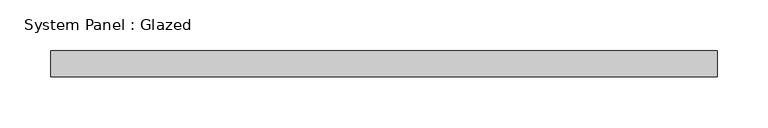
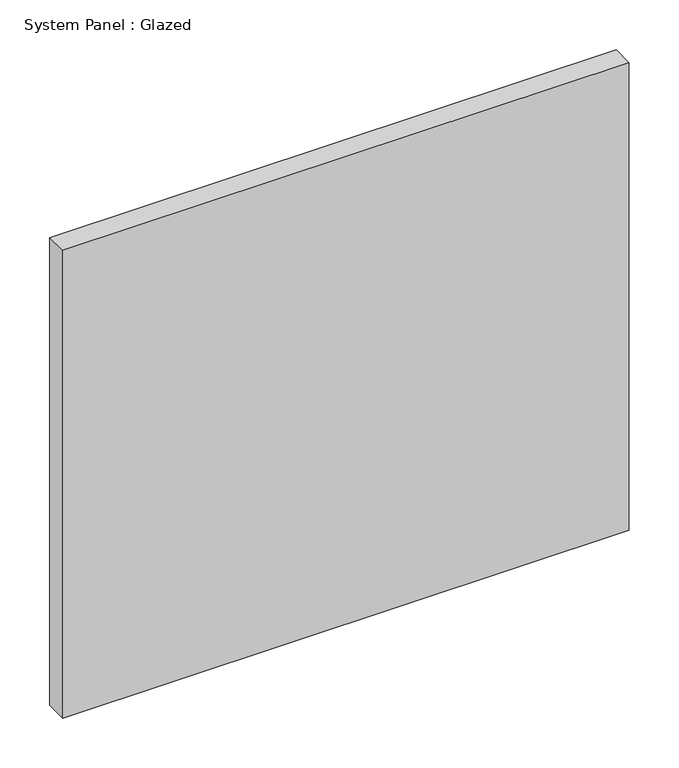
"""IFC4 building model written with IfcOpenShell, lengths in millimetres: plate geometry, System Panel : Glazed."""

from ifc_helpers import new_model, si_unit, origin, origin_with_axes, place, context, project, spatial, polyline, outline, extrude, source, transform, mapped, element, save


def system_panel_glazed_6e301024(model_context):
    return source(origin(), model_context, "Body", "SweptSolid", [
        extrude(outline(polyline([(327.3201314, 19.05), (-327.3201314, 19.05), (-327.3201314, 44.45), (327.3201314, 44.45), (327.3201314, 19.05)])), origin_with_axes(), (0.0, 0.0, 1.0), 571.5),
    ])


if __name__ == "__main__":
    model = new_model("IFC4")
    model_context = context("Model", 3, world=origin())
    ifc_project = project(units=[si_unit("LENGTHUNIT", "METRE", prefix="MILLI")], contexts=[model_context])
    site = spatial("IfcSite", under=ifc_project)
    building = spatial("IfcBuilding", under=site)
    placement = place(None, origin())
    system_panel_glazed_shape = system_panel_glazed_6e301024(model_context)
    element("IfcPlate", 1, ObjectType="System Panel : Glazed", at=placement, inside=building, context=model_context, shape_type="MappedRepresentation", body=[
        mapped(system_panel_glazed_shape, transform((0.0, 0.0, 0.0), x_axis=(1.0, 0.0, 0.0), y_axis=(0.0, 1.0, 0.0), z_axis=(0.0, 0.0, 1.0))),
    ])
    save(model, "model.ifc")

# Revit data of these elements
# Type "System Panel : Glazed"
#   Construction Type Id = "GSP4R"
#   Analytic Construction = "1/8 in Pilkington single glazing"
#   Visual Light Transmittance = 0.9
#   Solar Heat Gain Coefficient = 0.86
#   Heat Transfer Coefficient (U) = 1.18115 BTU/(h·ft²·°F)
#   Define Thermal Properties by = 1
# Element 1 (IfcPlate, "System Panel : Glazed")
#   Materials on its faces: "Glass"
# Materials
#   "Glass": class "Glass", colour RGB 0 128 192, transparency 0.75, Description = "Soda Lime Glass", Cost = 0
